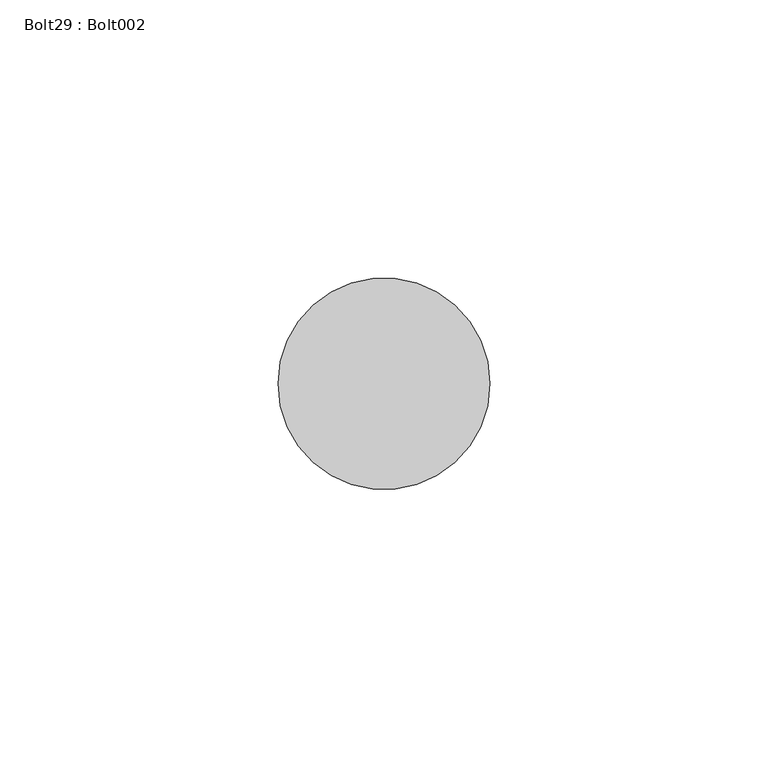
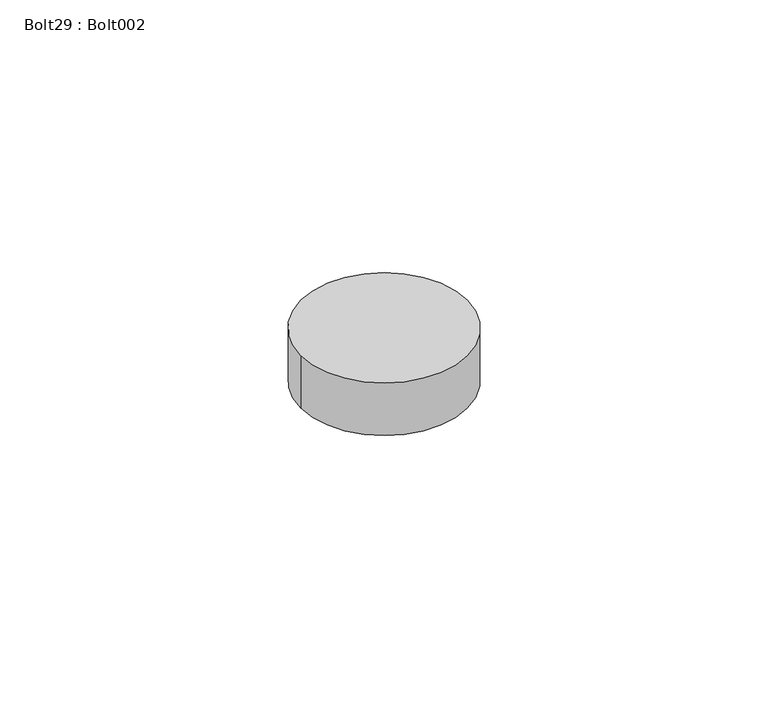
"""IFC4 building model written with IfcOpenShell, lengths in millimetres: proxy geometry, Bolt29 : Bolt002."""

from ifc_helpers import new_model, si_unit, point, frame, frame_2d, origin, place, context, project, spatial, circle_curve, trimmed, segment, composite_curve, outline, extrude, source, transform, mapped, element, save


def bolt29_bolt002_9d08b1a9(model_context):
    return source(origin(), model_context, "Body", "SweptSolid", [
        extrude(outline(composite_curve([segment(trimmed(circle_curve(frame_2d((5172.3828124, 1998.1882072)), 19.05), [point((5153.3328124, 1998.1882072))], [point((5191.4328124, 1998.1882072))], False, "CARTESIAN"), True, "CONTINUOUS"), segment(trimmed(circle_curve(frame_2d((5172.3828124, 1998.1882072)), 19.05), [point((5191.4328124, 1998.1882072))], [point((5153.3328124, 1998.1882072))], False, "CARTESIAN"), True, "CONTINUOUS")], self_intersect=False)), frame((0.0, 0.0, 36709.0959962), z_axis=(0.0, 0.0, 1.0), x_axis=(1.0, 0.0, 0.0)), (0.0, 0.0, 1.0), 12.7),
    ])


if __name__ == "__main__":
    model = new_model("IFC4")
    model_context = context("Model", 3, world=origin())
    ifc_project = project(units=[si_unit("LENGTHUNIT", "METRE", prefix="MILLI")], contexts=[model_context])
    site = spatial("IfcSite", under=ifc_project)
    building = spatial("IfcBuilding", under=site)
    placement = place(None, origin())
    bolt29_bolt002_shape = bolt29_bolt002_9d08b1a9(model_context)
    element("IfcBuildingElementProxy", 1, Name="Bolt29 : Bolt002", ObjectType="Bolt29 : Bolt002", at=placement, inside=building, context=model_context, shape_type="MappedRepresentation", body=[
        mapped(bolt29_bolt002_shape, transform((0.0, 0.0, 0.0), x_axis=(1.0, 0.0, 0.0), y_axis=(0.0, 1.0, 0.0), z_axis=(0.0, 0.0, 1.0))),
    ])
    save(model, "model.ifc")

# Revit data of these elements
# Type "Bolt29 : Bolt002"
#   NameOverride = "Bolt002"
# Element 1 (IfcBuildingElementProxy, "Bolt29 : Bolt002")
#   Materials on its faces: "STEEL ANGLE AND ANCHOR BOLT (SEE STRUCT. DWGS)"
# Materials
#   "STEEL ANGLE AND ANCHOR BOLT (SEE STRUCT. DWGS)": class "Unassigned", colour RGB 128 128 128, transparency 0, Cost = 0
